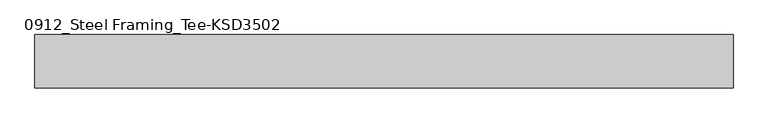
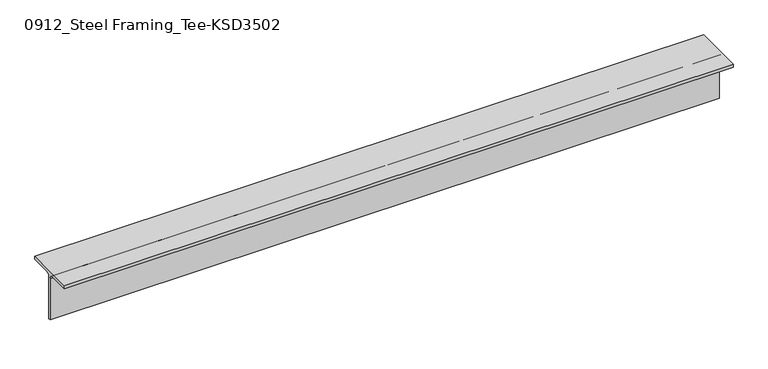
"""IFC4 building model written with IfcOpenShell, lengths in millimetres: member geometry, 0912_Steel Framing_Tee-KSD3502 : H_SB_ASB_CT-150x150x6.5x9."""

from ifc_helpers import new_model, si_unit, point, frame, frame_2d, origin, place, context, project, spatial, polyline, circle_curve, trimmed, segment, composite_curve, outline, extrude, source, transform, mapped, element, save


def member_0912_steel_framing_tee_ksd3502_3ebaf7cf(model_context):
    return source(origin(), model_context, "Body", "SweptSolid", [
        extrude(outline(composite_curve([segment(polyline([(75.0, 75.0), (75.0, 66.0), (16.25, 66.0)]), True, "CONTINUOUS"), segment(trimmed(circle_curve(frame_2d((16.25, 53.0)), 13.0), [point((16.25, 66.0))], [point((3.25, 53.0))], True, "CARTESIAN"), True, "CONTINUOUS"), segment(polyline([(3.25, 53.0), (3.25, -75.0), (-3.25, -75.0), (-3.25, 53.0)]), True, "CONTINUOUS"), segment(trimmed(circle_curve(frame_2d((-16.25, 53.0)), 13.0), [point((-3.25, 53.0))], [point((-16.25, 66.0))], True, "CARTESIAN"), True, "CONTINUOUS"), segment(polyline([(-16.25, 66.0), (-75.0, 66.0), (-75.0, 75.0), (75.0, 75.0)]), True, "CONTINUOUS")], self_intersect=False)), frame((-1124.25, 0.0, 0.0), z_axis=(1.0, 0.0, 0.0), x_axis=(0.0, 1.0, 0.0)), (0.0, 0.0, 1.0), 1966.5),
    ])


if __name__ == "__main__":
    model = new_model("IFC4")
    model_context = context("Model", 3, world=origin())
    ifc_project = project(units=[si_unit("LENGTHUNIT", "METRE", prefix="MILLI")], contexts=[model_context])
    site = spatial("IfcSite", under=ifc_project)
    building = spatial("IfcBuilding", under=site)
    placement = place(None, origin())
    member_0912_steel_framing_tee_ksd3502_shape = member_0912_steel_framing_tee_ksd3502_3ebaf7cf(model_context)
    element("IfcMember", 1, ObjectType="0912_Steel Framing_Tee-KSD3502 : H_SB_ASB_CT-150x150x6.5x9", at=placement, inside=building, context=model_context, shape_type="MappedRepresentation", body=[
        mapped(member_0912_steel_framing_tee_ksd3502_shape, transform((0.0, 0.0, 0.0), x_axis=(1.0, 0.0, 0.0), y_axis=(0.0, 1.0, 0.0), z_axis=(0.0, 0.0, 1.0))),
    ])
    save(model, "model.ifc")

# Revit data of these elements
# Type "0912_Steel Framing_Tee-KSD3502 : H_SB_ASB_CT-150x150x6.5x9"
#   H_WM Code_1 = "S01AA003-00001 | Main Steel Structure Fabrication Work | Shelter/Building | Light Steel - Standard (30KG/M>Weight) | Material: (   )"
#   H_WM Code_2 = "S03AA029-00001 | Main Steel Structure Erection Work | Shelter/Building | Light Steel (30KG/M>Weight) | Material: (   )"
#   H_WM Code_3 = "S01AA010-00001 | Main Steel Structure Fabrication Work | Shelter/Building | Steel Painting/Coating | for Non-Fireproofed Steel Surface, Surface Preparation, Primer, Second & Final Coat | Material: (   )"
#   H_Q'ty Cal Type Tag = "SB-Q2"
#   Width = 15.0 cm
#   Web Thickness = 0.65 cm
#   Web Fillet = 1.3 cm
#   Section Area = 23.39 cm²
#   Perimeter = 0.60 m²/m
#   Nominal Weight = 18.40 kgf/m
#   Height = 15.0 cm
#   Flange Thickness = 0.9 cm
#   Centroid Vertical = 7.5 cm
#   Centroid Horizontal = 7.5 cm
#   Length [instance default] = 1.5000 m
#   Structural Material [instance default] = Steel, 45-345
#   Warping Constant = (empty or 0)
#   Torsional Moment of Inertia = 0
#   Section Name Key = ""
#   Plastic Modulus weak axis = 0
#   Plastic Modulus strong axis = 0
#   Moment of Inertia weak axis = 0
#   Moment of Inertia strong axis = 0
#   Elastic Modulus weak axis = 0
#   Elastic Modulus strong axis = 0
#   Bolt Spacing = 0
#   Assembly Code = ""
# Element 1 (IfcMember, "0912_Steel Framing_Tee-KSD3502 : H_SB_ASB_CT-150x150x6.5x9")
#   Structural Material = none
# Materials
#   "Steel, 45-345": class "Metal", colour RGB 189 187 185, transparency 0, Description = "Steel 345 MPa", Cost = 0
